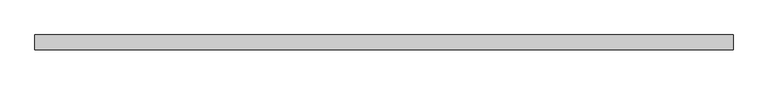
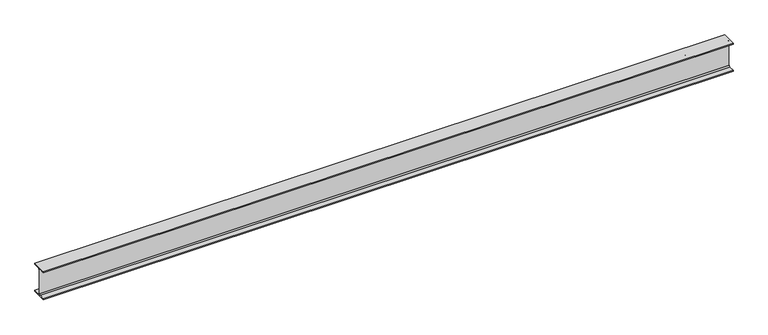
"""IFC4 building model written with IfcOpenShell, lengths in millimetres: beam geometry, 0912_Steel Framing_H-KSD3502 : H_SB_ASB_H-350x175x7x11."""

import ifcopenshell
import ifcopenshell.guid

model = None  # the IFC model being written
_history = None  # IfcOwnerHistory: only IFC2X3 demands one
_inside = {}  # id of a spatial element -> (the spatial element, [elements in it])
_under = {}  # id of a project, library or spatial element -> (it, [spatial elements below it])
_declared = {}  # id of a project -> (the project, [libraries it declares])
_typed = {}  # id of a type object -> (the type object, [elements of that type])
_made_of = {}  # id of a material, layer set ... -> (it, [elements and type objects made of it])


def new_model(schema):
    """Start an empty IFC model of exactly this schema.

    Asked for "IFC4X3", IfcOpenShell would pick the latest addendum, in which some entities
    have other attributes; the version numbers below select the first issue.
    IFC2X3 requires an IfcOwnerHistory on every rooted entity: one is made here for all.
    """
    global model, _history
    if schema == "IFC4X3":
        model = ifcopenshell.file(schema_version=(4, 3, 0, 0))
    else:
        model = ifcopenshell.file(schema=schema)
    _inside.clear()
    _under.clear()
    _declared.clear()
    _typed.clear()
    _made_of.clear()
    _history = None
    if model.schema == "IFC2X3":
        org = make("IfcOrganization", Name="unknown")
        user = make(
            "IfcPersonAndOrganization",
            ThePerson=make("IfcPerson", FamilyName="unknown"),
            TheOrganization=org,
        )
        app = make(
            "IfcApplication",
            ApplicationDeveloper=org,
            Version="unknown",
            ApplicationFullName="unknown",
            ApplicationIdentifier="unknown",
        )
        _history = make(
            "IfcOwnerHistory",
            OwningUser=user,
            OwningApplication=app,
            ChangeAction="ADDED",
            CreationDate=0,
        )
    return model


def make(cls, **values):
    """One entity of the class cls with the attributes given. An attribute that is None is left unset."""
    return model.create_entity(
        cls, **{name: value for name, value in values.items() if value is not None}
    )


def rooted(cls, **values):
    """An entity with a GlobalId (a new one), such as an element, a storey or a relation."""
    return make(cls, GlobalId=ifcopenshell.guid.new(), OwnerHistory=_history, **values)


def si_unit(unit_type, name, prefix=None):
    """IfcSIUnit, for example si_unit("LENGTHUNIT", "METRE", prefix="MILLI")."""
    return make("IfcSIUnit", UnitType=unit_type, Prefix=prefix, Name=name)


def assignment(units):
    """IfcUnitAssignment: the units of a project."""
    return None if units is None else make("IfcUnitAssignment", Units=units)


def point(xyz):
    """IfcCartesianPoint."""
    return None if xyz is None else make("IfcCartesianPoint", Coordinates=xyz)


def direction(xyz):
    """IfcDirection."""
    return None if xyz is None else make("IfcDirection", DirectionRatios=xyz)


def frame(location, z_axis=None, x_axis=None):
    """IfcAxis2Placement3D, a coordinate frame: its origin and axes. An axis left out is left unset."""
    return make(
        "IfcAxis2Placement3D",
        Location=point(location),
        Axis=direction(z_axis),
        RefDirection=direction(x_axis),
    )


def frame_2d(location, x_axis=None):
    """IfcAxis2Placement2D, a coordinate frame in the plane: its origin and x axis."""
    return make(
        "IfcAxis2Placement2D", Location=point(location), RefDirection=direction(x_axis)
    )


def origin():
    """The frame at (0, 0, 0) with its axes left unset."""
    return frame((0.0, 0.0, 0.0))


def place(relative_to, where):
    """IfcLocalPlacement: puts the frame where relative to a parent placement (None: the world)."""
    return make(
        "IfcLocalPlacement", PlacementRelTo=relative_to, RelativePlacement=where
    )


def context(
    kind, dimensions, precision=None, world=None, true_north=None, identifier=None
):
    """IfcGeometricRepresentationContext, for example the 3D "Model" context."""
    return make(
        "IfcGeometricRepresentationContext",
        ContextIdentifier=identifier,
        ContextType=kind,
        CoordinateSpaceDimension=dimensions,
        Precision=precision,
        WorldCoordinateSystem=world,
        TrueNorth=true_north,
    )


def project(units=None, contexts=None):
    """IfcProject with its units and contexts."""
    return rooted(
        "IfcProject",
        Name="project",
        RepresentationContexts=contexts,
        UnitsInContext=assignment(units),
    )


def spatial(cls, under=None, at=None, **own):
    """A site, building, storey or space (cls), placed at a placement, below another one or the project."""
    s = rooted(cls, ObjectPlacement=at, **own)
    if under is not None:
        _under.setdefault(under.id(), (under, []))[1].append(s)
    return s


def polyline(points):
    """IfcPolyline through the points."""
    return make("IfcPolyline", Points=[point(p) for p in points])


def circle_curve(where, radius):
    """IfcCircle in the frame where."""
    return make("IfcCircle", Position=where, Radius=radius)


def trimmed(basis, trim1, trim2, sense, master):
    """IfcTrimmedCurve: the piece of a basis curve between two trims."""
    return make(
        "IfcTrimmedCurve",
        BasisCurve=basis,
        Trim1=trim1,
        Trim2=trim2,
        SenseAgreement=sense,
        MasterRepresentation=master,
    )


def segment(curve, same_sense, transition):
    """IfcCompositeCurveSegment."""
    return make(
        "IfcCompositeCurveSegment",
        Transition=transition,
        SameSense=same_sense,
        ParentCurve=curve,
    )


def composite_curve(segments, self_intersect=None):
    """IfcCompositeCurve: segments joined end to end."""
    return make("IfcCompositeCurve", Segments=segments, SelfIntersect=self_intersect)


def outline(outer, holes=None, kind="AREA"):
    """IfcArbitraryClosedProfileDef: a profile drawn as a closed curve; with holes, ...WithVoids."""
    if holes is None:
        return make("IfcArbitraryClosedProfileDef", ProfileType=kind, OuterCurve=outer)
    return make(
        "IfcArbitraryProfileDefWithVoids",
        ProfileType=kind,
        OuterCurve=outer,
        InnerCurves=holes,
    )


def extrude(swept, where, along, depth):
    """IfcExtrudedAreaSolid: the profile swept, set in the frame where, extruded along a direction by depth."""
    return make(
        "IfcExtrudedAreaSolid",
        SweptArea=swept,
        Position=where,
        ExtrudedDirection=direction(along),
        Depth=depth,
    )


def shape(context_of_items, identifier, shape_type, items):
    """IfcShapeRepresentation: the items that make up one representation, for example the "Body"."""
    return make(
        "IfcShapeRepresentation",
        ContextOfItems=context_of_items,
        RepresentationIdentifier=identifier,
        RepresentationType=shape_type,
        Items=items,
    )


def source(mapping_origin, context_of_items, identifier, shape_type, items):
    """IfcRepresentationMap: a shape defined once, which mapped items show again and again."""
    return make(
        "IfcRepresentationMap",
        MappingOrigin=mapping_origin,
        MappedRepresentation=shape(context_of_items, identifier, shape_type, items),
    )


def transform(
    local_origin,
    x_axis=None,
    y_axis=None,
    z_axis=None,
    scale=None,
    scale2=None,
    scale3=None,
    uniform=True,
):
    """IfcCartesianTransformationOperator3D, or its non-uniform kind. x_axis, y_axis, z_axis: its Axis1, 2, 3."""
    if uniform:
        return make(
            "IfcCartesianTransformationOperator3D",
            Axis1=direction(x_axis),
            Axis2=direction(y_axis),
            LocalOrigin=point(local_origin),
            Scale=scale,
            Axis3=direction(z_axis),
        )
    return make(
        "IfcCartesianTransformationOperator3DnonUniform",
        Axis1=direction(x_axis),
        Axis2=direction(y_axis),
        LocalOrigin=point(local_origin),
        Scale=scale,
        Axis3=direction(z_axis),
        Scale2=scale2,
        Scale3=scale3,
    )


def mapped(mapping_source, mapping_target):
    """IfcMappedItem: shows the shape of a source again, moved by a transform."""
    return make(
        "IfcMappedItem", MappingSource=mapping_source, MappingTarget=mapping_target
    )


def made_of(thing, what):
    """Note that an element or type object is made of a material, layer set ...; save() writes the relation."""
    if what is not None:
        _made_of.setdefault(what.id(), (what, []))[1].append(thing)
    return thing


def element(
    cls,
    number,
    at=None,
    inside=None,
    cuts=None,
    type_object=None,
    material=None,
    context=None,
    identifier="Body",
    shape_type=None,
    held_by="IfcProductDefinitionShape",
    body=None,
    shapes=None,
    **own,
):
    """One element of the class cls, such as IfcWall. Its Tag is "e" and its number.

    at: its placement. inside: the storey or other place that contains it. cuts: it is an
    opening in that element (IfcRelVoidsElement). A single representation is given by context,
    identifier, shape_type and body (its items); several are given by shapes. held_by: the class
    of the entity that holds the representations. save() writes the other relations.
    """
    e = rooted(cls, Tag="e%d" % number, ObjectPlacement=at, **own)
    if body is not None:
        shapes = [shape(context, identifier, shape_type, body)]
    if shapes is not None:
        e.Representation = make(held_by, Representations=shapes)
    if inside is not None:
        _inside.setdefault(inside.id(), (inside, []))[1].append(e)
    if cuts is not None:
        rooted(
            "IfcRelVoidsElement", RelatingBuildingElement=cuts, RelatedOpeningElement=e
        )
    if type_object is not None:
        _typed.setdefault(type_object.id(), (type_object, []))[1].append(e)
    return made_of(e, material)


def aggregate(whole, parts):
    """IfcRelAggregates: a whole, such as a stair, and the parts it consists of."""
    return rooted("IfcRelAggregates", RelatingObject=whole, RelatedObjects=parts)


def save(model, path):
    """Write the relations noted so far, then the file.

    IfcRelAggregates (storeys below a building ...), IfcRelContainedInSpatialStructure (elements
    in a storey), IfcRelDefinesByType, IfcRelAssociatesMaterial and IfcRelDeclares: one each for
    every whole, place, type object, material and project.
    """
    for whole, parts in _under.values():
        aggregate(whole, parts)
    for where, things in _inside.values():
        rooted(
            "IfcRelContainedInSpatialStructure",
            RelatedElements=things,
            RelatingStructure=where,
        )
    for kind, things in _typed.values():
        rooted("IfcRelDefinesByType", RelatedObjects=things, RelatingType=kind)
    for what, things in _made_of.values():
        rooted("IfcRelAssociatesMaterial", RelatedObjects=things, RelatingMaterial=what)
    for by, libraries in _declared.values():
        rooted("IfcRelDeclares", RelatingContext=by, RelatedDefinitions=libraries)
    model.write(path)


def beam_11403a9d(model_context):
    return source(origin(), model_context, "Body", "SweptSolid", [
        extrude(outline(composite_curve([segment(polyline([(87.5, -164.0), (87.5, -175.0), (-87.5, -175.0), (-87.5, -164.0), (-17.5, -164.0)]), True, "CONTINUOUS"), segment(trimmed(circle_curve(frame_2d((-17.5, -150.0)), 14.0), [point((-17.5, -164.0))], [point((-3.5, -150.0))], True, "CARTESIAN"), True, "CONTINUOUS"), segment(polyline([(-3.5, -150.0), (-3.5, 150.0)]), True, "CONTINUOUS"), segment(trimmed(circle_curve(frame_2d((-17.5, 150.0)), 14.0), [point((-3.5, 150.0))], [point((-17.5, 164.0))], True, "CARTESIAN"), True, "CONTINUOUS"), segment(polyline([(-17.5, 164.0), (-87.5, 164.0), (-87.5, 175.0), (87.5, 175.0), (87.5, 164.0), (17.5, 164.0)]), True, "CONTINUOUS"), segment(trimmed(circle_curve(frame_2d((17.5, 150.0)), 14.0), [point((17.5, 164.0))], [point((3.5, 150.0))], True, "CARTESIAN"), True, "CONTINUOUS"), segment(polyline([(3.5, 150.0), (3.5, -150.0)]), True, "CONTINUOUS"), segment(trimmed(circle_curve(frame_2d((17.5, -150.0)), 14.0), [point((3.5, -150.0))], [point((17.5, -164.0))], True, "CARTESIAN"), True, "CONTINUOUS"), segment(polyline([(17.5, -164.0), (87.5, -164.0)]), True, "CONTINUOUS")], self_intersect=False)), frame((-4087.3, 0.0, 0.0), z_axis=(1.0, 0.0, 0.0), x_axis=(0.0, 1.0, 0.0)), (0.0, 0.0, 1.0), 8174.6),
    ])


if __name__ == "__main__":
    model = new_model("IFC4")
    model_context = context("Model", 3, world=origin())
    ifc_project = project(units=[si_unit("LENGTHUNIT", "METRE", prefix="MILLI")], contexts=[model_context])
    site = spatial("IfcSite", under=ifc_project)
    building = spatial("IfcBuilding", under=site)
    placement = place(None, origin())
    beam_shape = beam_11403a9d(model_context)
    element("IfcBeam", 1, ObjectType="0912_Steel Framing_H-KSD3502 : H_SB_ASB_H-350x175x7x11", at=placement, inside=building, context=model_context, shape_type="MappedRepresentation", body=[
        mapped(beam_shape, transform((0.0, 0.0, 0.0), x_axis=(1.0, 0.0, 0.0), y_axis=(0.0, 1.0, 0.0), z_axis=(0.0, 0.0, 1.0))),
    ])
    save(model, "model.ifc")

# Revit data of these elements
# Type "0912_Steel Framing_H-KSD3502 : H_SB_ASB_H-350x175x7x11"
#   H_WM Code_1 = "S01AA002-00001 | Main Steel Structure Fabrication Work | Shelter/Building | Medium Steel - Standard (90KG/M>Weight≥30KG/M) | Material: (   )"
#   H_WM Code_2 = "S03AA028-00001 | Main Steel Structure Erection Work | Shelter/Building | Medium Steel (90KG/M>Weight≥30KG/M) | Material: (   )"
#   H_WM Code_3 = "S01AA010-00001 | Main Steel Structure Fabrication Work | Shelter/Building | Steel Painting/Coating | for Non-Fireproofed Steel Surface, Surface Preparation, Primer, Second & Final Coat | Material: (   )"
#   H_Q'ty Cal Type Tag = "SB-Q2"
#   Width = 17.5 cm
#   Web Thickness = 0.7 cm
#   Web Fillet = 1.4 cm
#   Warping Constant = 282000.0 cm⁶
#   W = 0
#   Torsional Moment of Inertia = 19.4042 cm⁴
#   Section Area = 63.14 cm²
#   Plastic Modulus weak axis = 174.0 cm³
#   Plastic Modulus strong axis = 868.0 cm³
#   Perimeter = 1.36 m²/m
#   Nominal Weight = 49.60 kgf/m
#   Moment of Inertia weak axis = 984.00 cm⁴
#   Moment of Inertia strong axis = 13600.00 cm⁴
#   Height = 35.0 cm
#   Flange Thickness = 1.1 cm
#   Elastic Modulus weak axis = 112.0 cm³
#   Elastic Modulus strong axis = 775.0 cm³
#   Centroid Vertical = 17.5 cm
#   Centroid Horizontal = 8.75 cm
#   Ix = 136000000
#   Length [instance default] = 1.5240 m
#   Zx = 868000
#   b = 0.1750 m
#   h = 0.3500 m
#   r = 0.0140 m
#   s = 0.0070 m
#   t = 0.0110 m
#   A = 0.006314 m²
#   Structural Material [instance default] = Steel, 45-345
#   Assembly Code = ""
# Element 1 (IfcBeam, "0912_Steel Framing_H-KSD3502 : H_SB_ASB_H-350x175x7x11")
#   Structural Material = none
# Materials
#   "Steel, 45-345": class "Metal", colour RGB 189 187 185, transparency 0, Description = "Steel 345 MPa", Cost = 0
